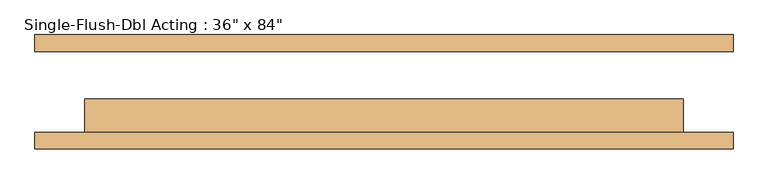
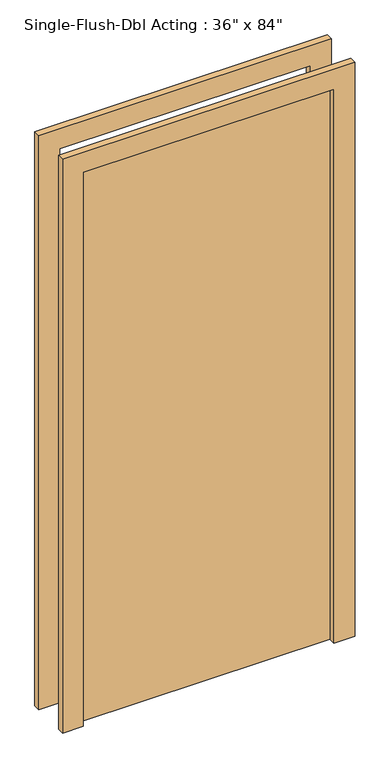
"""IFC4 building model written with IfcOpenShell, lengths in millimetres: door geometry."""

import ifcopenshell
import ifcopenshell.guid

model = None  # the IFC model being written
_history = None  # IfcOwnerHistory: only IFC2X3 demands one
_inside = {}  # id of a spatial element -> (the spatial element, [elements in it])
_under = {}  # id of a project, library or spatial element -> (it, [spatial elements below it])
_declared = {}  # id of a project -> (the project, [libraries it declares])
_typed = {}  # id of a type object -> (the type object, [elements of that type])
_made_of = {}  # id of a material, layer set ... -> (it, [elements and type objects made of it])


def new_model(schema):
    """Start an empty IFC model of exactly this schema.

    Asked for "IFC4X3", IfcOpenShell would pick the latest addendum, in which some entities
    have other attributes; the version numbers below select the first issue.
    IFC2X3 requires an IfcOwnerHistory on every rooted entity: one is made here for all.
    """
    global model, _history
    if schema == "IFC4X3":
        model = ifcopenshell.file(schema_version=(4, 3, 0, 0))
    else:
        model = ifcopenshell.file(schema=schema)
    _inside.clear()
    _under.clear()
    _declared.clear()
    _typed.clear()
    _made_of.clear()
    _history = None
    if model.schema == "IFC2X3":
        org = make("IfcOrganization", Name="unknown")
        user = make(
            "IfcPersonAndOrganization",
            ThePerson=make("IfcPerson", FamilyName="unknown"),
            TheOrganization=org,
        )
        app = make(
            "IfcApplication",
            ApplicationDeveloper=org,
            Version="unknown",
            ApplicationFullName="unknown",
            ApplicationIdentifier="unknown",
        )
        _history = make(
            "IfcOwnerHistory",
            OwningUser=user,
            OwningApplication=app,
            ChangeAction="ADDED",
            CreationDate=0,
        )
    return model


def make(cls, **values):
    """One entity of the class cls with the attributes given. An attribute that is None is left unset."""
    return model.create_entity(
        cls, **{name: value for name, value in values.items() if value is not None}
    )


def rooted(cls, **values):
    """An entity with a GlobalId (a new one), such as an element, a storey or a relation."""
    return make(cls, GlobalId=ifcopenshell.guid.new(), OwnerHistory=_history, **values)


def si_unit(unit_type, name, prefix=None):
    """IfcSIUnit, for example si_unit("LENGTHUNIT", "METRE", prefix="MILLI")."""
    return make("IfcSIUnit", UnitType=unit_type, Prefix=prefix, Name=name)


def assignment(units):
    """IfcUnitAssignment: the units of a project."""
    return None if units is None else make("IfcUnitAssignment", Units=units)


def point(xyz):
    """IfcCartesianPoint."""
    return None if xyz is None else make("IfcCartesianPoint", Coordinates=xyz)


def direction(xyz):
    """IfcDirection."""
    return None if xyz is None else make("IfcDirection", DirectionRatios=xyz)


def frame(location, z_axis=None, x_axis=None):
    """IfcAxis2Placement3D, a coordinate frame: its origin and axes. An axis left out is left unset."""
    return make(
        "IfcAxis2Placement3D",
        Location=point(location),
        Axis=direction(z_axis),
        RefDirection=direction(x_axis),
    )


def origin():
    """The frame at (0, 0, 0) with its axes left unset."""
    return frame((0.0, 0.0, 0.0))


def origin_with_axes():
    """The frame at (0, 0, 0) with the z axis (0, 0, 1) and the x axis (1, 0, 0) written out."""
    return frame((0.0, 0.0, 0.0), z_axis=(0.0, 0.0, 1.0), x_axis=(1.0, 0.0, 0.0))


def place(relative_to, where):
    """IfcLocalPlacement: puts the frame where relative to a parent placement (None: the world)."""
    return make(
        "IfcLocalPlacement", PlacementRelTo=relative_to, RelativePlacement=where
    )


def context(
    kind, dimensions, precision=None, world=None, true_north=None, identifier=None
):
    """IfcGeometricRepresentationContext, for example the 3D "Model" context."""
    return make(
        "IfcGeometricRepresentationContext",
        ContextIdentifier=identifier,
        ContextType=kind,
        CoordinateSpaceDimension=dimensions,
        Precision=precision,
        WorldCoordinateSystem=world,
        TrueNorth=true_north,
    )


def project(units=None, contexts=None):
    """IfcProject with its units and contexts."""
    return rooted(
        "IfcProject",
        Name="project",
        RepresentationContexts=contexts,
        UnitsInContext=assignment(units),
    )


def spatial(cls, under=None, at=None, **own):
    """A site, building, storey or space (cls), placed at a placement, below another one or the project."""
    s = rooted(cls, ObjectPlacement=at, **own)
    if under is not None:
        _under.setdefault(under.id(), (under, []))[1].append(s)
    return s


def polyline(points):
    """IfcPolyline through the points."""
    return make("IfcPolyline", Points=[point(p) for p in points])


def outline(outer, holes=None, kind="AREA"):
    """IfcArbitraryClosedProfileDef: a profile drawn as a closed curve; with holes, ...WithVoids."""
    if holes is None:
        return make("IfcArbitraryClosedProfileDef", ProfileType=kind, OuterCurve=outer)
    return make(
        "IfcArbitraryProfileDefWithVoids",
        ProfileType=kind,
        OuterCurve=outer,
        InnerCurves=holes,
    )


def extrude(swept, where, along, depth):
    """IfcExtrudedAreaSolid: the profile swept, set in the frame where, extruded along a direction by depth."""
    return make(
        "IfcExtrudedAreaSolid",
        SweptArea=swept,
        Position=where,
        ExtrudedDirection=direction(along),
        Depth=depth,
    )


def shape(context_of_items, identifier, shape_type, items):
    """IfcShapeRepresentation: the items that make up one representation, for example the "Body"."""
    return make(
        "IfcShapeRepresentation",
        ContextOfItems=context_of_items,
        RepresentationIdentifier=identifier,
        RepresentationType=shape_type,
        Items=items,
    )


def source(mapping_origin, context_of_items, identifier, shape_type, items):
    """IfcRepresentationMap: a shape defined once, which mapped items show again and again."""
    return make(
        "IfcRepresentationMap",
        MappingOrigin=mapping_origin,
        MappedRepresentation=shape(context_of_items, identifier, shape_type, items),
    )


def transform(
    local_origin,
    x_axis=None,
    y_axis=None,
    z_axis=None,
    scale=None,
    scale2=None,
    scale3=None,
    uniform=True,
):
    """IfcCartesianTransformationOperator3D, or its non-uniform kind. x_axis, y_axis, z_axis: its Axis1, 2, 3."""
    if uniform:
        return make(
            "IfcCartesianTransformationOperator3D",
            Axis1=direction(x_axis),
            Axis2=direction(y_axis),
            LocalOrigin=point(local_origin),
            Scale=scale,
            Axis3=direction(z_axis),
        )
    return make(
        "IfcCartesianTransformationOperator3DnonUniform",
        Axis1=direction(x_axis),
        Axis2=direction(y_axis),
        LocalOrigin=point(local_origin),
        Scale=scale,
        Axis3=direction(z_axis),
        Scale2=scale2,
        Scale3=scale3,
    )


def mapped(mapping_source, mapping_target):
    """IfcMappedItem: shows the shape of a source again, moved by a transform."""
    return make(
        "IfcMappedItem", MappingSource=mapping_source, MappingTarget=mapping_target
    )


def made_of(thing, what):
    """Note that an element or type object is made of a material, layer set ...; save() writes the relation."""
    if what is not None:
        _made_of.setdefault(what.id(), (what, []))[1].append(thing)
    return thing


def element(
    cls,
    number,
    at=None,
    inside=None,
    cuts=None,
    type_object=None,
    material=None,
    context=None,
    identifier="Body",
    shape_type=None,
    held_by="IfcProductDefinitionShape",
    body=None,
    shapes=None,
    **own,
):
    """One element of the class cls, such as IfcWall. Its Tag is "e" and its number.

    at: its placement. inside: the storey or other place that contains it. cuts: it is an
    opening in that element (IfcRelVoidsElement). A single representation is given by context,
    identifier, shape_type and body (its items); several are given by shapes. held_by: the class
    of the entity that holds the representations. save() writes the other relations.
    """
    e = rooted(cls, Tag="e%d" % number, ObjectPlacement=at, **own)
    if body is not None:
        shapes = [shape(context, identifier, shape_type, body)]
    if shapes is not None:
        e.Representation = make(held_by, Representations=shapes)
    if inside is not None:
        _inside.setdefault(inside.id(), (inside, []))[1].append(e)
    if cuts is not None:
        rooted(
            "IfcRelVoidsElement", RelatingBuildingElement=cuts, RelatedOpeningElement=e
        )
    if type_object is not None:
        _typed.setdefault(type_object.id(), (type_object, []))[1].append(e)
    return made_of(e, material)


def aggregate(whole, parts):
    """IfcRelAggregates: a whole, such as a stair, and the parts it consists of."""
    return rooted("IfcRelAggregates", RelatingObject=whole, RelatedObjects=parts)


def save(model, path):
    """Write the relations noted so far, then the file.

    IfcRelAggregates (storeys below a building ...), IfcRelContainedInSpatialStructure (elements
    in a storey), IfcRelDefinesByType, IfcRelAssociatesMaterial and IfcRelDeclares: one each for
    every whole, place, type object, material and project.
    """
    for whole, parts in _under.values():
        aggregate(whole, parts)
    for where, things in _inside.values():
        rooted(
            "IfcRelContainedInSpatialStructure",
            RelatedElements=things,
            RelatingStructure=where,
        )
    for kind, things in _typed.values():
        rooted("IfcRelDefinesByType", RelatedObjects=things, RelatingType=kind)
    for what, things in _made_of.values():
        rooted("IfcRelAssociatesMaterial", RelatedObjects=things, RelatingMaterial=what)
    for by, libraries in _declared.values():
        rooted("IfcRelDeclares", RelatingContext=by, RelatedDefinitions=libraries)
    model.write(path)


def door_eb9f8b14(model_context):
    return source(origin(), model_context, "Body", "SweptSolid", [
        extrude(outline(polyline([(2209.8, -533.4), (0.0, -533.4), (0.0, -457.2), (2133.6, -457.2), (2133.6, 457.2), (0.0, 457.2), (0.0, 533.4), (2209.8, 533.4), (2209.8, -533.4)])), frame((0.0, -87.3125, 0.0), z_axis=(0.0, 1.0, 0.0), x_axis=(0.0, 0.0, 1.0)), (0.0, 0.0, 1.0), 25.4),
        extrude(outline(polyline([(2209.8, 533.4), (2209.8, -533.4), (0.0, -533.4), (0.0, -457.2), (2133.6, -457.2), (2133.6, 457.2), (0.0, 457.2), (0.0, 533.4), (2209.8, 533.4)])), frame((0.0, 61.9125, 0.0), z_axis=(0.0, 1.0, 0.0), x_axis=(0.0, 0.0, 1.0)), (0.0, 0.0, 1.0), 25.4),
        extrude(outline(polyline([(457.2, -11.1125), (457.2, -61.9125), (-457.2, -61.9125), (-457.2, -11.1125), (457.2, -11.1125)])), origin_with_axes(), (0.0, 0.0, 1.0), 2133.6),
    ])


if __name__ == "__main__":
    model = new_model("IFC4")
    model_context = context("Model", 3, world=origin())
    ifc_project = project(units=[si_unit("LENGTHUNIT", "METRE", prefix="MILLI")], contexts=[model_context])
    site = spatial("IfcSite", under=ifc_project)
    building = spatial("IfcBuilding", under=site)
    placement = place(None, origin())
    door_shape = door_eb9f8b14(model_context)
    element("IfcDoor", 1, ObjectType="Single-Flush-Dbl Acting : 36\" x 84\"", at=placement, inside=building, context=model_context, shape_type="MappedRepresentation", body=[
        mapped(door_shape, transform((0.0, 0.0, 0.0), x_axis=(1.0, 0.0, 0.0), y_axis=(0.0, 1.0, 0.0), z_axis=(0.0, 0.0, 1.0))),
    ])
    save(model, "model.ifc")

# Revit data of these elements
# Project information
#   Room Abbreviation = "ORSR1"
#   Room Description = "Sterile Processing, Surgical Services (ORSR1)"
#   Sheets - Total = "5"
#   Project Issue Date = "Issue Date"
#   Project Status = "Project Status"
#   Client Name = "Owner"
#   Project Address = "Enter address here"
#   Project Name = "Project Name"
#   Project Number = "Project Number"
#   Publication Date = "30-Jan-15"
# Type "Single-Flush-Dbl Acting : 36\" x 84\""
#   Type Mark = "10"
#   Assembly Code = "C1020"
#   Thickness = 0' - 2"
#   Height = 7' - 0"
#   Rail Width - Center = 0' - 4"
#   Trim Projection Ext. = 0' - 1"
#   Trim Projection Int. = 0' - 1"
#   Trim Width Ext. = 0' - 3"
#   Trim Width Int. = 0' - 3"
#   Width = 3' - 0"
#   Door Material = Door - Panel
#   Frame Material = Door - Frame
#   Function = (empty or 0)
#   Construction Type = (empty or 0)
#   Wall Closure = (empty or 0)
# Element 1 (IfcDoor, "Single-Flush-Dbl Acting : 36\" x 84\"")
#   Materials on its faces: "Door - Frame", "Door - Panel"
# Materials
#   "Door - Panel": class "Wood", colour RGB 210 159 95, transparency 0
#   "Door - Frame": class "Miscellaneous", colour RGB 118 70 51, transparency 0
